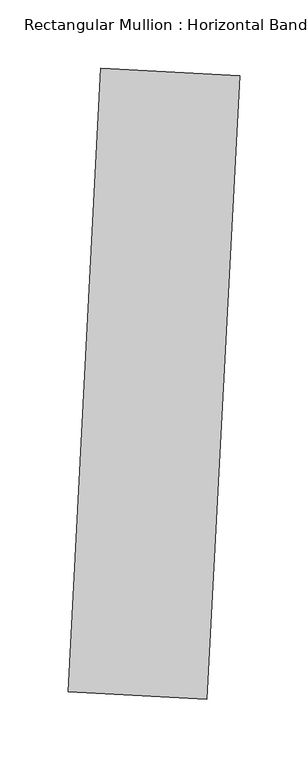
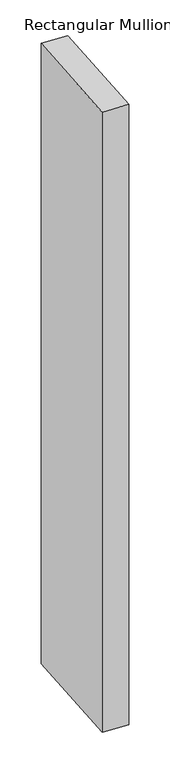
"""IFC4 building model written with IfcOpenShell, lengths in millimetres: member geometry, Rectangular Mullion : Horizontal Band."""

import ifcopenshell
import ifcopenshell.guid

model = None  # the IFC model being written
_history = None  # IfcOwnerHistory: only IFC2X3 demands one
_inside = {}  # id of a spatial element -> (the spatial element, [elements in it])
_under = {}  # id of a project, library or spatial element -> (it, [spatial elements below it])
_declared = {}  # id of a project -> (the project, [libraries it declares])
_typed = {}  # id of a type object -> (the type object, [elements of that type])
_made_of = {}  # id of a material, layer set ... -> (it, [elements and type objects made of it])


def new_model(schema):
    """Start an empty IFC model of exactly this schema.

    Asked for "IFC4X3", IfcOpenShell would pick the latest addendum, in which some entities
    have other attributes; the version numbers below select the first issue.
    IFC2X3 requires an IfcOwnerHistory on every rooted entity: one is made here for all.
    """
    global model, _history
    if schema == "IFC4X3":
        model = ifcopenshell.file(schema_version=(4, 3, 0, 0))
    else:
        model = ifcopenshell.file(schema=schema)
    _inside.clear()
    _under.clear()
    _declared.clear()
    _typed.clear()
    _made_of.clear()
    _history = None
    if model.schema == "IFC2X3":
        org = make("IfcOrganization", Name="unknown")
        user = make(
            "IfcPersonAndOrganization",
            ThePerson=make("IfcPerson", FamilyName="unknown"),
            TheOrganization=org,
        )
        app = make(
            "IfcApplication",
            ApplicationDeveloper=org,
            Version="unknown",
            ApplicationFullName="unknown",
            ApplicationIdentifier="unknown",
        )
        _history = make(
            "IfcOwnerHistory",
            OwningUser=user,
            OwningApplication=app,
            ChangeAction="ADDED",
            CreationDate=0,
        )
    return model


def make(cls, **values):
    """One entity of the class cls with the attributes given. An attribute that is None is left unset."""
    return model.create_entity(
        cls, **{name: value for name, value in values.items() if value is not None}
    )


def rooted(cls, **values):
    """An entity with a GlobalId (a new one), such as an element, a storey or a relation."""
    return make(cls, GlobalId=ifcopenshell.guid.new(), OwnerHistory=_history, **values)


def si_unit(unit_type, name, prefix=None):
    """IfcSIUnit, for example si_unit("LENGTHUNIT", "METRE", prefix="MILLI")."""
    return make("IfcSIUnit", UnitType=unit_type, Prefix=prefix, Name=name)


def assignment(units):
    """IfcUnitAssignment: the units of a project."""
    return None if units is None else make("IfcUnitAssignment", Units=units)


def point(xyz):
    """IfcCartesianPoint."""
    return None if xyz is None else make("IfcCartesianPoint", Coordinates=xyz)


def direction(xyz):
    """IfcDirection."""
    return None if xyz is None else make("IfcDirection", DirectionRatios=xyz)


def frame(location, z_axis=None, x_axis=None):
    """IfcAxis2Placement3D, a coordinate frame: its origin and axes. An axis left out is left unset."""
    return make(
        "IfcAxis2Placement3D",
        Location=point(location),
        Axis=direction(z_axis),
        RefDirection=direction(x_axis),
    )


def origin():
    """The frame at (0, 0, 0) with its axes left unset."""
    return frame((0.0, 0.0, 0.0))


def place(relative_to, where):
    """IfcLocalPlacement: puts the frame where relative to a parent placement (None: the world)."""
    return make(
        "IfcLocalPlacement", PlacementRelTo=relative_to, RelativePlacement=where
    )


def context(
    kind, dimensions, precision=None, world=None, true_north=None, identifier=None
):
    """IfcGeometricRepresentationContext, for example the 3D "Model" context."""
    return make(
        "IfcGeometricRepresentationContext",
        ContextIdentifier=identifier,
        ContextType=kind,
        CoordinateSpaceDimension=dimensions,
        Precision=precision,
        WorldCoordinateSystem=world,
        TrueNorth=true_north,
    )


def project(units=None, contexts=None):
    """IfcProject with its units and contexts."""
    return rooted(
        "IfcProject",
        Name="project",
        RepresentationContexts=contexts,
        UnitsInContext=assignment(units),
    )


def spatial(cls, under=None, at=None, **own):
    """A site, building, storey or space (cls), placed at a placement, below another one or the project."""
    s = rooted(cls, ObjectPlacement=at, **own)
    if under is not None:
        _under.setdefault(under.id(), (under, []))[1].append(s)
    return s


def polyline(points):
    """IfcPolyline through the points."""
    return make("IfcPolyline", Points=[point(p) for p in points])


def outline(outer, holes=None, kind="AREA"):
    """IfcArbitraryClosedProfileDef: a profile drawn as a closed curve; with holes, ...WithVoids."""
    if holes is None:
        return make("IfcArbitraryClosedProfileDef", ProfileType=kind, OuterCurve=outer)
    return make(
        "IfcArbitraryProfileDefWithVoids",
        ProfileType=kind,
        OuterCurve=outer,
        InnerCurves=holes,
    )


def extrude(swept, where, along, depth):
    """IfcExtrudedAreaSolid: the profile swept, set in the frame where, extruded along a direction by depth."""
    return make(
        "IfcExtrudedAreaSolid",
        SweptArea=swept,
        Position=where,
        ExtrudedDirection=direction(along),
        Depth=depth,
    )


def shape(context_of_items, identifier, shape_type, items):
    """IfcShapeRepresentation: the items that make up one representation, for example the "Body"."""
    return make(
        "IfcShapeRepresentation",
        ContextOfItems=context_of_items,
        RepresentationIdentifier=identifier,
        RepresentationType=shape_type,
        Items=items,
    )


def source(mapping_origin, context_of_items, identifier, shape_type, items):
    """IfcRepresentationMap: a shape defined once, which mapped items show again and again."""
    return make(
        "IfcRepresentationMap",
        MappingOrigin=mapping_origin,
        MappedRepresentation=shape(context_of_items, identifier, shape_type, items),
    )


def transform(
    local_origin,
    x_axis=None,
    y_axis=None,
    z_axis=None,
    scale=None,
    scale2=None,
    scale3=None,
    uniform=True,
):
    """IfcCartesianTransformationOperator3D, or its non-uniform kind. x_axis, y_axis, z_axis: its Axis1, 2, 3."""
    if uniform:
        return make(
            "IfcCartesianTransformationOperator3D",
            Axis1=direction(x_axis),
            Axis2=direction(y_axis),
            LocalOrigin=point(local_origin),
            Scale=scale,
            Axis3=direction(z_axis),
        )
    return make(
        "IfcCartesianTransformationOperator3DnonUniform",
        Axis1=direction(x_axis),
        Axis2=direction(y_axis),
        LocalOrigin=point(local_origin),
        Scale=scale,
        Axis3=direction(z_axis),
        Scale2=scale2,
        Scale3=scale3,
    )


def mapped(mapping_source, mapping_target):
    """IfcMappedItem: shows the shape of a source again, moved by a transform."""
    return make(
        "IfcMappedItem", MappingSource=mapping_source, MappingTarget=mapping_target
    )


def made_of(thing, what):
    """Note that an element or type object is made of a material, layer set ...; save() writes the relation."""
    if what is not None:
        _made_of.setdefault(what.id(), (what, []))[1].append(thing)
    return thing


def element(
    cls,
    number,
    at=None,
    inside=None,
    cuts=None,
    type_object=None,
    material=None,
    context=None,
    identifier="Body",
    shape_type=None,
    held_by="IfcProductDefinitionShape",
    body=None,
    shapes=None,
    **own,
):
    """One element of the class cls, such as IfcWall. Its Tag is "e" and its number.

    at: its placement. inside: the storey or other place that contains it. cuts: it is an
    opening in that element (IfcRelVoidsElement). A single representation is given by context,
    identifier, shape_type and body (its items); several are given by shapes. held_by: the class
    of the entity that holds the representations. save() writes the other relations.
    """
    e = rooted(cls, Tag="e%d" % number, ObjectPlacement=at, **own)
    if body is not None:
        shapes = [shape(context, identifier, shape_type, body)]
    if shapes is not None:
        e.Representation = make(held_by, Representations=shapes)
    if inside is not None:
        _inside.setdefault(inside.id(), (inside, []))[1].append(e)
    if cuts is not None:
        rooted(
            "IfcRelVoidsElement", RelatingBuildingElement=cuts, RelatedOpeningElement=e
        )
    if type_object is not None:
        _typed.setdefault(type_object.id(), (type_object, []))[1].append(e)
    return made_of(e, material)


def aggregate(whole, parts):
    """IfcRelAggregates: a whole, such as a stair, and the parts it consists of."""
    return rooted("IfcRelAggregates", RelatingObject=whole, RelatedObjects=parts)


def save(model, path):
    """Write the relations noted so far, then the file.

    IfcRelAggregates (storeys below a building ...), IfcRelContainedInSpatialStructure (elements
    in a storey), IfcRelDefinesByType, IfcRelAssociatesMaterial and IfcRelDeclares: one each for
    every whole, place, type object, material and project.
    """
    for whole, parts in _under.values():
        aggregate(whole, parts)
    for where, things in _inside.values():
        rooted(
            "IfcRelContainedInSpatialStructure",
            RelatedElements=things,
            RelatingStructure=where,
        )
    for kind, things in _typed.values():
        rooted("IfcRelDefinesByType", RelatedObjects=things, RelatingType=kind)
    for what, things in _made_of.values():
        rooted("IfcRelAssociatesMaterial", RelatedObjects=things, RelatingMaterial=what)
    for by, libraries in _declared.values():
        rooted("IfcRelDeclares", RelatingContext=by, RelatedDefinitions=libraries)
    model.write(path)


def rectangular_mullion_horizontal_band_466c517c(model_context):
    return source(origin(), model_context, "Body", "SweptSolid", [
        extrude(outline(polyline([(62.69438, 301.8280451), (38.7663808, -154.7453782), (-62.69438, -149.4280451), (-38.7663808, 307.1453782), (62.69438, 301.8280451)])), frame((0.0, 0.0, -2573.7181637), z_axis=(0.0, 0.0, 1.0), x_axis=(1.0, 0.0, 0.0)), (0.0, 0.0, 1.0), 2573.7181637),
    ])


if __name__ == "__main__":
    model = new_model("IFC4")
    model_context = context("Model", 3, world=origin())
    ifc_project = project(units=[si_unit("LENGTHUNIT", "METRE", prefix="MILLI")], contexts=[model_context])
    site = spatial("IfcSite", under=ifc_project)
    building = spatial("IfcBuilding", under=site)
    placement = place(None, origin())
    rectangular_mullion_horizontal_band_shape = rectangular_mullion_horizontal_band_466c517c(model_context)
    element("IfcMember", 1, ObjectType="Rectangular Mullion : Horizontal Band", at=placement, inside=building, context=model_context, shape_type="MappedRepresentation", body=[
        mapped(rectangular_mullion_horizontal_band_shape, transform((0.0, 0.0, 0.0), x_axis=(1.0, 0.0, 0.0), y_axis=(0.0, 1.0, 0.0), z_axis=(0.0, 0.0, 1.0))),
    ])
    save(model, "model.ifc")

# Revit data of these elements
# Type "Rectangular Mullion : Horizontal Band"
#   built-in parameter 1007351 = 0.25 (stored number, unit not read)
#   built-in parameter 1007304 = 1.5 (stored number, unit not read)
#   built-in parameter 1007301 = 0.166667 (stored number, unit not read)
#   built-in parameter 1007300 = 0.166667 (stored number, unit not read)
# Element 1 (IfcMember, "Rectangular Mullion : Horizontal Band")
#   Materials on its faces: "Aluminum"
# Materials
#   "Aluminum": class "Metal", colour RGB 247 247 247, transparency 0, Description = "Aluminum 6061", Cost = 0
